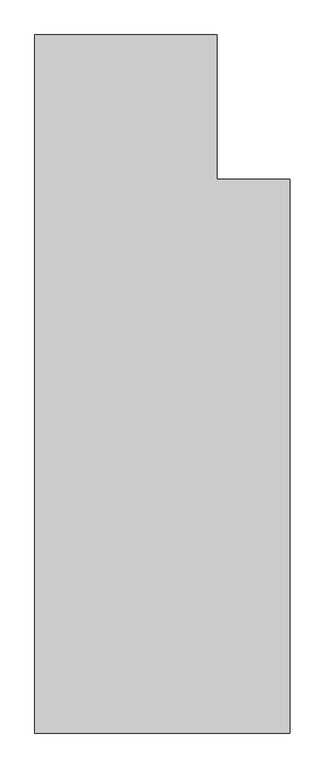
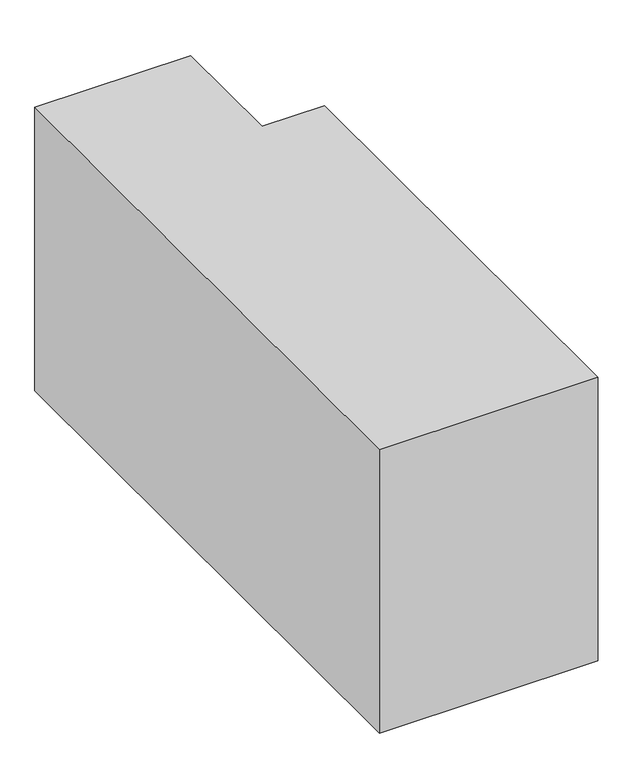
"""IFC4 building model written with IfcOpenShell, lengths in millimetres: proxy geometry, 0_3d."""

from ifc_helpers import new_model, si_unit, origin, origin_with_axes, place, context, project, spatial, polyline, outline, extrude, source, transform, mapped, element, save


def generic_models_364c7734(model_context):
    return source(origin(), model_context, "Body", "SweptSolid", [
        extrude(outline(polyline([(2100.0, 0.0), (0.0, 0.0), (0.0, 5742.0), (1500.0, 5742.0), (1500.0, 4553.8742346), (2100.0, 4553.8742346), (2100.0, 0.0)])), origin_with_axes(), (0.0, 0.0, 1.0), 2880.0),
    ])


if __name__ == "__main__":
    model = new_model("IFC4")
    model_context = context("Model", 3, world=origin())
    ifc_project = project(units=[si_unit("LENGTHUNIT", "METRE", prefix="MILLI")], contexts=[model_context])
    site = spatial("IfcSite", under=ifc_project)
    building = spatial("IfcBuilding", under=site)
    placement = place(None, origin())
    generic_models_shape = generic_models_364c7734(model_context)
    element("IfcBuildingElementProxy", 1, Name="0_3d", ObjectType="0_3d", at=placement, inside=building, context=model_context, shape_type="MappedRepresentation", body=[
        mapped(generic_models_shape, transform((0.0, 0.0, 0.0), x_axis=(1.0, 0.0, 0.0), y_axis=(0.0, 1.0, 0.0), z_axis=(0.0, 0.0, 1.0))),
    ])
    save(model, "model.ifc")

# Revit data of these elements
# Element 1 (IfcBuildingElementProxy, "0_3d")
#   Materials on its faces: "*1"
# Materials
#   "*1": class "Unassigned", colour RGB 175 175 175, transparency 0
